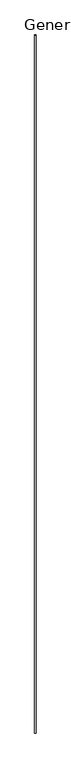
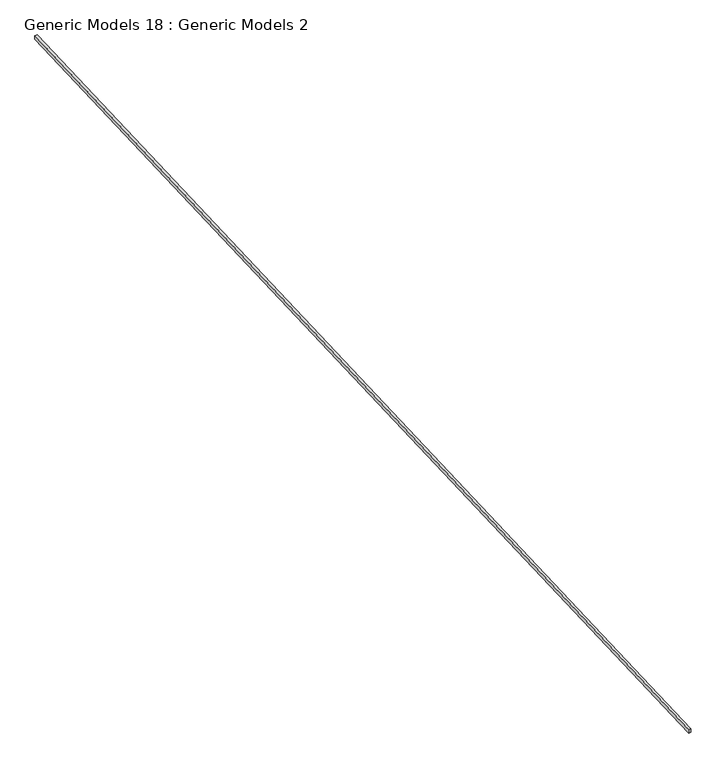
"""IFC4 building model written with IfcOpenShell, lengths in millimetres: proxy geometry, Generic Models 18 : Generic Models 2."""

from ifc_helpers import new_model, si_unit, frame, origin, place, context, project, spatial, polyline, outline, extrude, source, transform, mapped, element, save


def generic_models_18_generic_models_2_a34fcc10(model_context):
    return source(origin(), model_context, "Body", "SweptSolid", [
        extrude(outline(polyline([(-62.0335059, 0.0), (-3.5113078, 0.0), (-3.5113078, -9.5782693), (5.4689483, -18.5585254), (5.4689483, -105.4094913), (-62.0335059, -105.4094913), (-62.0335059, 0.0)])), frame((667612.9591395, -569870.0067055, 8700.9626568), z_axis=(0.0, 0.9991330730923521, 0.041630544712176844), x_axis=(1.0, 0.0, 0.0)), (0.0, 0.0, 1.0), 33312.3541237),
    ])


if __name__ == "__main__":
    model = new_model("IFC4")
    model_context = context("Model", 3, world=origin())
    ifc_project = project(units=[si_unit("LENGTHUNIT", "METRE", prefix="MILLI")], contexts=[model_context])
    site = spatial("IfcSite", under=ifc_project)
    building = spatial("IfcBuilding", under=site)
    placement = place(None, origin())
    generic_models_18_generic_models_2_shape = generic_models_18_generic_models_2_a34fcc10(model_context)
    element("IfcBuildingElementProxy", 1, Name="Generic Models 18 : Generic Models 2", ObjectType="Generic Models 18 : Generic Models 2", at=placement, inside=building, context=model_context, shape_type="MappedRepresentation", body=[
        mapped(generic_models_18_generic_models_2_shape, transform((0.0, 0.0, 0.0), x_axis=(1.0, 0.0, 0.0), y_axis=(0.0, 1.0, 0.0), z_axis=(0.0, 0.0, 1.0))),
    ])
    save(model, "model.ifc")

# Revit data of these elements
# Element 1 (IfcBuildingElementProxy, "Generic Models 18 : Generic Models 2")
#   Materials on its faces: "LOW VOLUMN EXPANDABLE FOAM INSULATION (CLASS A FLAME SPREAD)"
# Materials
#   "LOW VOLUMN EXPANDABLE FOAM INSULATION (CLASS A FLAME SPREAD)": class "Unassigned", colour RGB 213 216 95, transparency 0, Cost = 0
